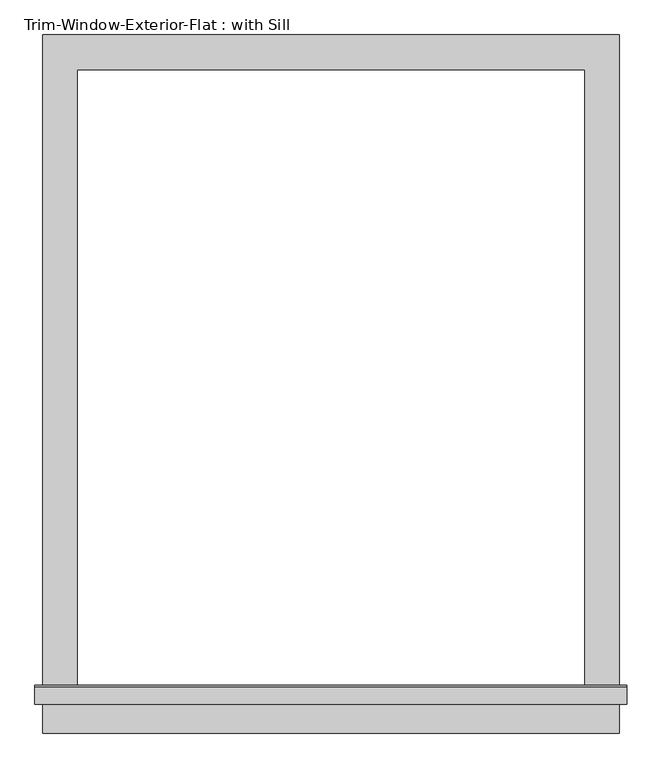
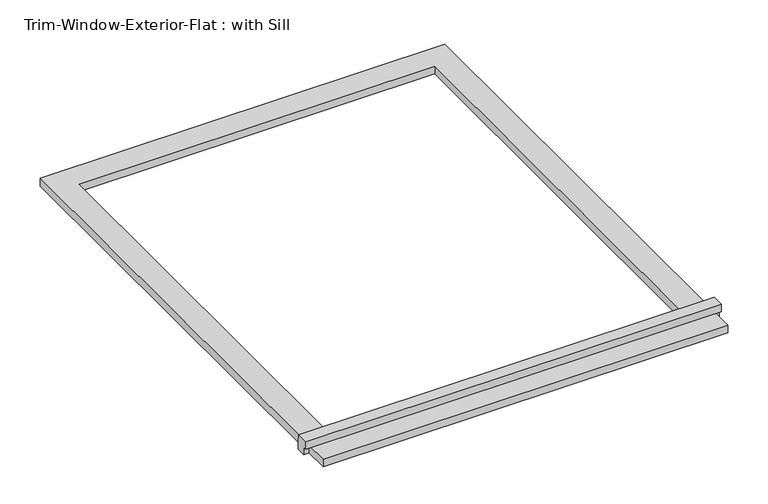
"""IFC4 building model written with IfcOpenShell, lengths in millimetres: proxy geometry, Trim-Window-Exterior-Flat : with Sill."""

import ifcopenshell
import ifcopenshell.guid

model = None  # the IFC model being written
_history = None  # IfcOwnerHistory: only IFC2X3 demands one
_inside = {}  # id of a spatial element -> (the spatial element, [elements in it])
_under = {}  # id of a project, library or spatial element -> (it, [spatial elements below it])
_declared = {}  # id of a project -> (the project, [libraries it declares])
_typed = {}  # id of a type object -> (the type object, [elements of that type])
_made_of = {}  # id of a material, layer set ... -> (it, [elements and type objects made of it])


def new_model(schema):
    """Start an empty IFC model of exactly this schema.

    Asked for "IFC4X3", IfcOpenShell would pick the latest addendum, in which some entities
    have other attributes; the version numbers below select the first issue.
    IFC2X3 requires an IfcOwnerHistory on every rooted entity: one is made here for all.
    """
    global model, _history
    if schema == "IFC4X3":
        model = ifcopenshell.file(schema_version=(4, 3, 0, 0))
    else:
        model = ifcopenshell.file(schema=schema)
    _inside.clear()
    _under.clear()
    _declared.clear()
    _typed.clear()
    _made_of.clear()
    _history = None
    if model.schema == "IFC2X3":
        org = make("IfcOrganization", Name="unknown")
        user = make(
            "IfcPersonAndOrganization",
            ThePerson=make("IfcPerson", FamilyName="unknown"),
            TheOrganization=org,
        )
        app = make(
            "IfcApplication",
            ApplicationDeveloper=org,
            Version="unknown",
            ApplicationFullName="unknown",
            ApplicationIdentifier="unknown",
        )
        _history = make(
            "IfcOwnerHistory",
            OwningUser=user,
            OwningApplication=app,
            ChangeAction="ADDED",
            CreationDate=0,
        )
    return model


def make(cls, **values):
    """One entity of the class cls with the attributes given. An attribute that is None is left unset."""
    return model.create_entity(
        cls, **{name: value for name, value in values.items() if value is not None}
    )


def rooted(cls, **values):
    """An entity with a GlobalId (a new one), such as an element, a storey or a relation."""
    return make(cls, GlobalId=ifcopenshell.guid.new(), OwnerHistory=_history, **values)


def si_unit(unit_type, name, prefix=None):
    """IfcSIUnit, for example si_unit("LENGTHUNIT", "METRE", prefix="MILLI")."""
    return make("IfcSIUnit", UnitType=unit_type, Prefix=prefix, Name=name)


def assignment(units):
    """IfcUnitAssignment: the units of a project."""
    return None if units is None else make("IfcUnitAssignment", Units=units)


def point(xyz):
    """IfcCartesianPoint."""
    return None if xyz is None else make("IfcCartesianPoint", Coordinates=xyz)


def direction(xyz):
    """IfcDirection."""
    return None if xyz is None else make("IfcDirection", DirectionRatios=xyz)


def frame(location, z_axis=None, x_axis=None):
    """IfcAxis2Placement3D, a coordinate frame: its origin and axes. An axis left out is left unset."""
    return make(
        "IfcAxis2Placement3D",
        Location=point(location),
        Axis=direction(z_axis),
        RefDirection=direction(x_axis),
    )


def origin():
    """The frame at (0, 0, 0) with its axes left unset."""
    return frame((0.0, 0.0, 0.0))


def origin_with_axes():
    """The frame at (0, 0, 0) with the z axis (0, 0, 1) and the x axis (1, 0, 0) written out."""
    return frame((0.0, 0.0, 0.0), z_axis=(0.0, 0.0, 1.0), x_axis=(1.0, 0.0, 0.0))


def place(relative_to, where):
    """IfcLocalPlacement: puts the frame where relative to a parent placement (None: the world)."""
    return make(
        "IfcLocalPlacement", PlacementRelTo=relative_to, RelativePlacement=where
    )


def context(
    kind, dimensions, precision=None, world=None, true_north=None, identifier=None
):
    """IfcGeometricRepresentationContext, for example the 3D "Model" context."""
    return make(
        "IfcGeometricRepresentationContext",
        ContextIdentifier=identifier,
        ContextType=kind,
        CoordinateSpaceDimension=dimensions,
        Precision=precision,
        WorldCoordinateSystem=world,
        TrueNorth=true_north,
    )


def project(units=None, contexts=None):
    """IfcProject with its units and contexts."""
    return rooted(
        "IfcProject",
        Name="project",
        RepresentationContexts=contexts,
        UnitsInContext=assignment(units),
    )


def spatial(cls, under=None, at=None, **own):
    """A site, building, storey or space (cls), placed at a placement, below another one or the project."""
    s = rooted(cls, ObjectPlacement=at, **own)
    if under is not None:
        _under.setdefault(under.id(), (under, []))[1].append(s)
    return s


def polyline(points):
    """IfcPolyline through the points."""
    return make("IfcPolyline", Points=[point(p) for p in points])


def outline(outer, holes=None, kind="AREA"):
    """IfcArbitraryClosedProfileDef: a profile drawn as a closed curve; with holes, ...WithVoids."""
    if holes is None:
        return make("IfcArbitraryClosedProfileDef", ProfileType=kind, OuterCurve=outer)
    return make(
        "IfcArbitraryProfileDefWithVoids",
        ProfileType=kind,
        OuterCurve=outer,
        InnerCurves=holes,
    )


def extrude(swept, where, along, depth):
    """IfcExtrudedAreaSolid: the profile swept, set in the frame where, extruded along a direction by depth."""
    return make(
        "IfcExtrudedAreaSolid",
        SweptArea=swept,
        Position=where,
        ExtrudedDirection=direction(along),
        Depth=depth,
    )


def shape(context_of_items, identifier, shape_type, items):
    """IfcShapeRepresentation: the items that make up one representation, for example the "Body"."""
    return make(
        "IfcShapeRepresentation",
        ContextOfItems=context_of_items,
        RepresentationIdentifier=identifier,
        RepresentationType=shape_type,
        Items=items,
    )


def source(mapping_origin, context_of_items, identifier, shape_type, items):
    """IfcRepresentationMap: a shape defined once, which mapped items show again and again."""
    return make(
        "IfcRepresentationMap",
        MappingOrigin=mapping_origin,
        MappedRepresentation=shape(context_of_items, identifier, shape_type, items),
    )


def transform(
    local_origin,
    x_axis=None,
    y_axis=None,
    z_axis=None,
    scale=None,
    scale2=None,
    scale3=None,
    uniform=True,
):
    """IfcCartesianTransformationOperator3D, or its non-uniform kind. x_axis, y_axis, z_axis: its Axis1, 2, 3."""
    if uniform:
        return make(
            "IfcCartesianTransformationOperator3D",
            Axis1=direction(x_axis),
            Axis2=direction(y_axis),
            LocalOrigin=point(local_origin),
            Scale=scale,
            Axis3=direction(z_axis),
        )
    return make(
        "IfcCartesianTransformationOperator3DnonUniform",
        Axis1=direction(x_axis),
        Axis2=direction(y_axis),
        LocalOrigin=point(local_origin),
        Scale=scale,
        Axis3=direction(z_axis),
        Scale2=scale2,
        Scale3=scale3,
    )


def mapped(mapping_source, mapping_target):
    """IfcMappedItem: shows the shape of a source again, moved by a transform."""
    return make(
        "IfcMappedItem", MappingSource=mapping_source, MappingTarget=mapping_target
    )


def made_of(thing, what):
    """Note that an element or type object is made of a material, layer set ...; save() writes the relation."""
    if what is not None:
        _made_of.setdefault(what.id(), (what, []))[1].append(thing)
    return thing


def element(
    cls,
    number,
    at=None,
    inside=None,
    cuts=None,
    type_object=None,
    material=None,
    context=None,
    identifier="Body",
    shape_type=None,
    held_by="IfcProductDefinitionShape",
    body=None,
    shapes=None,
    **own,
):
    """One element of the class cls, such as IfcWall. Its Tag is "e" and its number.

    at: its placement. inside: the storey or other place that contains it. cuts: it is an
    opening in that element (IfcRelVoidsElement). A single representation is given by context,
    identifier, shape_type and body (its items); several are given by shapes. held_by: the class
    of the entity that holds the representations. save() writes the other relations.
    """
    e = rooted(cls, Tag="e%d" % number, ObjectPlacement=at, **own)
    if body is not None:
        shapes = [shape(context, identifier, shape_type, body)]
    if shapes is not None:
        e.Representation = make(held_by, Representations=shapes)
    if inside is not None:
        _inside.setdefault(inside.id(), (inside, []))[1].append(e)
    if cuts is not None:
        rooted(
            "IfcRelVoidsElement", RelatingBuildingElement=cuts, RelatedOpeningElement=e
        )
    if type_object is not None:
        _typed.setdefault(type_object.id(), (type_object, []))[1].append(e)
    return made_of(e, material)


def aggregate(whole, parts):
    """IfcRelAggregates: a whole, such as a stair, and the parts it consists of."""
    return rooted("IfcRelAggregates", RelatingObject=whole, RelatedObjects=parts)


def save(model, path):
    """Write the relations noted so far, then the file.

    IfcRelAggregates (storeys below a building ...), IfcRelContainedInSpatialStructure (elements
    in a storey), IfcRelDefinesByType, IfcRelAssociatesMaterial and IfcRelDeclares: one each for
    every whole, place, type object, material and project.
    """
    for whole, parts in _under.values():
        aggregate(whole, parts)
    for where, things in _inside.values():
        rooted(
            "IfcRelContainedInSpatialStructure",
            RelatedElements=things,
            RelatingStructure=where,
        )
    for kind, things in _typed.values():
        rooted("IfcRelDefinesByType", RelatedObjects=things, RelatingType=kind)
    for what, things in _made_of.values():
        rooted("IfcRelAssociatesMaterial", RelatedObjects=things, RelatingMaterial=what)
    for by, libraries in _declared.values():
        rooted("IfcRelDeclares", RelatingContext=by, RelatedDefinitions=libraries)
    model.write(path)


def trim_window_exterior_flat_with_sill_d0c475a0(model_context):
    return source(origin(), model_context, "Body", "SweptSolid", [
        extrude(outline(polyline([(476.25, -1038.1823709), (476.25, -1095.3323709), (-476.25, -1095.3323709), (-476.25, -1038.1823709), (476.25, -1038.1823709)])), origin_with_axes(), (0.0, 0.0, 1.0), 19.05),
        extrude(outline(polyline([(-1047.75, 38.1), (-1018.4580645, 38.1), (-1016.0, 19.05), (-1016.0, 0.0), (-1038.1823709, 0.0), (-1038.1823709, 19.05), (-1047.75, 19.05), (-1047.75, 38.1)])), frame((-488.95, 0.0, 0.0), z_axis=(1.0, 0.0, 0.0), x_axis=(0.0, 1.0, 0.0)), (0.0, 0.0, 1.0), 977.9),
        extrude(outline(polyline([(-476.25, 57.15), (476.25, 57.15), (476.25, -1016.0), (419.1, -1016.0), (419.1, 0.0), (-419.1, 0.0), (-419.1, -1016.0), (-476.25, -1016.0), (-476.25, 57.15)])), origin_with_axes(), (0.0, 0.0, 1.0), 19.05),
    ])


if __name__ == "__main__":
    model = new_model("IFC4")
    model_context = context("Model", 3, world=origin())
    ifc_project = project(units=[si_unit("LENGTHUNIT", "METRE", prefix="MILLI")], contexts=[model_context])
    site = spatial("IfcSite", under=ifc_project)
    building = spatial("IfcBuilding", under=site)
    placement = place(None, origin())
    trim_window_exterior_flat_with_sill_shape = trim_window_exterior_flat_with_sill_d0c475a0(model_context)
    element("IfcBuildingElementProxy", 1, Name="Trim-Window-Exterior-Flat : with Sill", ObjectType="Trim-Window-Exterior-Flat : with Sill", at=placement, inside=building, context=model_context, shape_type="MappedRepresentation", body=[
        mapped(trim_window_exterior_flat_with_sill_shape, transform((0.0, 0.0, 0.0), x_axis=(1.0, 0.0, 0.0), y_axis=(0.0, 1.0, 0.0), z_axis=(0.0, 0.0, 1.0))),
    ])
    save(model, "model.ifc")

# Revit data of these elements
# Type "Trim-Window-Exterior-Flat : with Sill"
#   Trim Width = 0' - 2 1/4"
#   Trim Thickness_Picture Frame = 0' - 1 1/4"
#   Trim Thickness_with Sill = 0' - 0 3/4"
#   Sill Thickness = 0' - 1 1/4"
#   Opening Width [instance default] = 2' - 0"
#   Opening Height [instance default] = 3' - 0"
#   Default Elevation = 4' - 0"
#   Sill = yes
#   Picture Frame = no
#   Trim Material [instance default] = none
# Element 1 (IfcBuildingElementProxy, "Trim-Window-Exterior-Flat : with Sill")
#   Opening Width = 2' - 9"
#   Opening Height = 3' - 4"
#   Trim Material = Clad - White
#   Materials on its faces: "Clad - White"
# Materials
#   "Clad - White": class "Wood", colour RGB 242 242 238, transparency 0, Cost = 0
